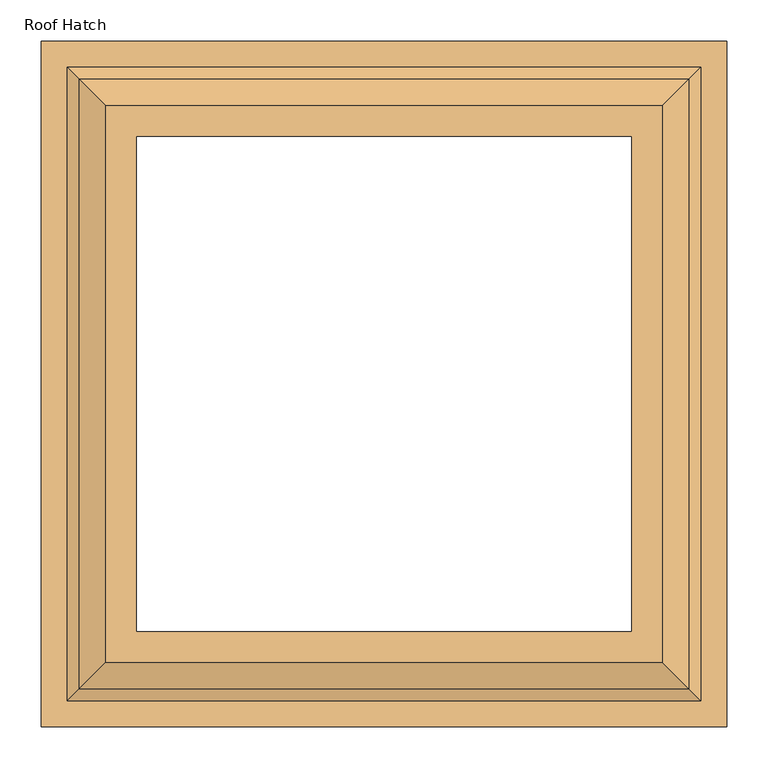
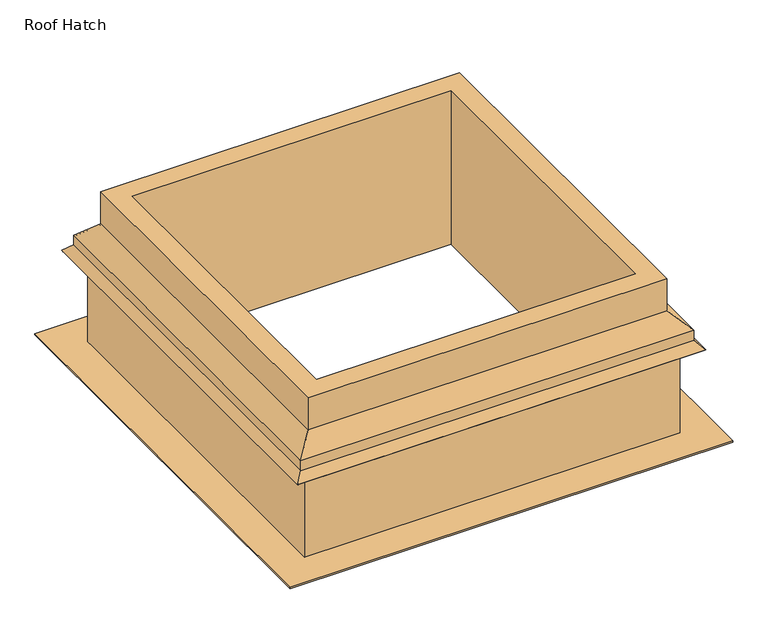
"""IFC4 building model written with IfcOpenShell, lengths in millimetres: door geometry, Alçap_o : Roof Hatch."""

import ifcopenshell
import ifcopenshell.guid

model = None  # the IFC model being written
_history = None  # IfcOwnerHistory: only IFC2X3 demands one
_inside = {}  # id of a spatial element -> (the spatial element, [elements in it])
_under = {}  # id of a project, library or spatial element -> (it, [spatial elements below it])
_declared = {}  # id of a project -> (the project, [libraries it declares])
_typed = {}  # id of a type object -> (the type object, [elements of that type])
_made_of = {}  # id of a material, layer set ... -> (it, [elements and type objects made of it])


def new_model(schema):
    """Start an empty IFC model of exactly this schema.

    Asked for "IFC4X3", IfcOpenShell would pick the latest addendum, in which some entities
    have other attributes; the version numbers below select the first issue.
    IFC2X3 requires an IfcOwnerHistory on every rooted entity: one is made here for all.
    """
    global model, _history
    if schema == "IFC4X3":
        model = ifcopenshell.file(schema_version=(4, 3, 0, 0))
    else:
        model = ifcopenshell.file(schema=schema)
    _inside.clear()
    _under.clear()
    _declared.clear()
    _typed.clear()
    _made_of.clear()
    _history = None
    if model.schema == "IFC2X3":
        org = make("IfcOrganization", Name="unknown")
        user = make(
            "IfcPersonAndOrganization",
            ThePerson=make("IfcPerson", FamilyName="unknown"),
            TheOrganization=org,
        )
        app = make(
            "IfcApplication",
            ApplicationDeveloper=org,
            Version="unknown",
            ApplicationFullName="unknown",
            ApplicationIdentifier="unknown",
        )
        _history = make(
            "IfcOwnerHistory",
            OwningUser=user,
            OwningApplication=app,
            ChangeAction="ADDED",
            CreationDate=0,
        )
    return model


def make(cls, **values):
    """One entity of the class cls with the attributes given. An attribute that is None is left unset."""
    return model.create_entity(
        cls, **{name: value for name, value in values.items() if value is not None}
    )


def rooted(cls, **values):
    """An entity with a GlobalId (a new one), such as an element, a storey or a relation."""
    return make(cls, GlobalId=ifcopenshell.guid.new(), OwnerHistory=_history, **values)


def si_unit(unit_type, name, prefix=None):
    """IfcSIUnit, for example si_unit("LENGTHUNIT", "METRE", prefix="MILLI")."""
    return make("IfcSIUnit", UnitType=unit_type, Prefix=prefix, Name=name)


def assignment(units):
    """IfcUnitAssignment: the units of a project."""
    return None if units is None else make("IfcUnitAssignment", Units=units)


def point(xyz):
    """IfcCartesianPoint."""
    return None if xyz is None else make("IfcCartesianPoint", Coordinates=xyz)


def direction(xyz):
    """IfcDirection."""
    return None if xyz is None else make("IfcDirection", DirectionRatios=xyz)


def frame(location, z_axis=None, x_axis=None):
    """IfcAxis2Placement3D, a coordinate frame: its origin and axes. An axis left out is left unset."""
    return make(
        "IfcAxis2Placement3D",
        Location=point(location),
        Axis=direction(z_axis),
        RefDirection=direction(x_axis),
    )


def origin():
    """The frame at (0, 0, 0) with its axes left unset."""
    return frame((0.0, 0.0, 0.0))


def place(relative_to, where):
    """IfcLocalPlacement: puts the frame where relative to a parent placement (None: the world)."""
    return make(
        "IfcLocalPlacement", PlacementRelTo=relative_to, RelativePlacement=where
    )


def context(
    kind, dimensions, precision=None, world=None, true_north=None, identifier=None
):
    """IfcGeometricRepresentationContext, for example the 3D "Model" context."""
    return make(
        "IfcGeometricRepresentationContext",
        ContextIdentifier=identifier,
        ContextType=kind,
        CoordinateSpaceDimension=dimensions,
        Precision=precision,
        WorldCoordinateSystem=world,
        TrueNorth=true_north,
    )


def project(units=None, contexts=None):
    """IfcProject with its units and contexts."""
    return rooted(
        "IfcProject",
        Name="project",
        RepresentationContexts=contexts,
        UnitsInContext=assignment(units),
    )


def spatial(cls, under=None, at=None, **own):
    """A site, building, storey or space (cls), placed at a placement, below another one or the project."""
    s = rooted(cls, ObjectPlacement=at, **own)
    if under is not None:
        _under.setdefault(under.id(), (under, []))[1].append(s)
    return s


def faces_of(points, faces, orient=None, outer=None):
    """IfcFace entities. A face is a list of loops; a loop is a list of indices into points, from 0.

    orient and outer hold one flag for each loop. By default every Orientation is true, the
    first loop of a face is its IfcFaceOuterBound and the others are IfcFaceBound.
    """
    made = []
    for i, loops in enumerate(faces):
        bounds = []
        for j, loop in enumerate(loops):
            is_outer = j == 0 if outer is None else outer[i][j]
            bounds.append(
                make(
                    "IfcFaceOuterBound" if is_outer else "IfcFaceBound",
                    Bound=make("IfcPolyLoop", Polygon=[points[k] for k in loop]),
                    Orientation=True if orient is None else orient[i][j],
                )
            )
        made.append(make("IfcFace", Bounds=bounds))
    return made


def faceted_brep(points, faces, orient=None, outer=None, voids=None):
    """IfcFacetedBrep: a solid bounded by flat faces; with voids (closed shells), ...WithVoids."""
    shared = [point(p) for p in points]
    hull = make("IfcClosedShell", CfsFaces=faces_of(shared, faces, orient, outer))
    if voids is None:
        return make("IfcFacetedBrep", Outer=hull)
    return make(
        "IfcFacetedBrepWithVoids",
        Outer=hull,
        Voids=[
            make(cls, CfsFaces=faces_of(shared, fs, o, b)) for cls, fs, o, b in voids
        ],
    )


def shape(context_of_items, identifier, shape_type, items):
    """IfcShapeRepresentation: the items that make up one representation, for example the "Body"."""
    return make(
        "IfcShapeRepresentation",
        ContextOfItems=context_of_items,
        RepresentationIdentifier=identifier,
        RepresentationType=shape_type,
        Items=items,
    )


def source(mapping_origin, context_of_items, identifier, shape_type, items):
    """IfcRepresentationMap: a shape defined once, which mapped items show again and again."""
    return make(
        "IfcRepresentationMap",
        MappingOrigin=mapping_origin,
        MappedRepresentation=shape(context_of_items, identifier, shape_type, items),
    )


def transform(
    local_origin,
    x_axis=None,
    y_axis=None,
    z_axis=None,
    scale=None,
    scale2=None,
    scale3=None,
    uniform=True,
):
    """IfcCartesianTransformationOperator3D, or its non-uniform kind. x_axis, y_axis, z_axis: its Axis1, 2, 3."""
    if uniform:
        return make(
            "IfcCartesianTransformationOperator3D",
            Axis1=direction(x_axis),
            Axis2=direction(y_axis),
            LocalOrigin=point(local_origin),
            Scale=scale,
            Axis3=direction(z_axis),
        )
    return make(
        "IfcCartesianTransformationOperator3DnonUniform",
        Axis1=direction(x_axis),
        Axis2=direction(y_axis),
        LocalOrigin=point(local_origin),
        Scale=scale,
        Axis3=direction(z_axis),
        Scale2=scale2,
        Scale3=scale3,
    )


def mapped(mapping_source, mapping_target):
    """IfcMappedItem: shows the shape of a source again, moved by a transform."""
    return make(
        "IfcMappedItem", MappingSource=mapping_source, MappingTarget=mapping_target
    )


def made_of(thing, what):
    """Note that an element or type object is made of a material, layer set ...; save() writes the relation."""
    if what is not None:
        _made_of.setdefault(what.id(), (what, []))[1].append(thing)
    return thing


def element(
    cls,
    number,
    at=None,
    inside=None,
    cuts=None,
    type_object=None,
    material=None,
    context=None,
    identifier="Body",
    shape_type=None,
    held_by="IfcProductDefinitionShape",
    body=None,
    shapes=None,
    **own,
):
    """One element of the class cls, such as IfcWall. Its Tag is "e" and its number.

    at: its placement. inside: the storey or other place that contains it. cuts: it is an
    opening in that element (IfcRelVoidsElement). A single representation is given by context,
    identifier, shape_type and body (its items); several are given by shapes. held_by: the class
    of the entity that holds the representations. save() writes the other relations.
    """
    e = rooted(cls, Tag="e%d" % number, ObjectPlacement=at, **own)
    if body is not None:
        shapes = [shape(context, identifier, shape_type, body)]
    if shapes is not None:
        e.Representation = make(held_by, Representations=shapes)
    if inside is not None:
        _inside.setdefault(inside.id(), (inside, []))[1].append(e)
    if cuts is not None:
        rooted(
            "IfcRelVoidsElement", RelatingBuildingElement=cuts, RelatedOpeningElement=e
        )
    if type_object is not None:
        _typed.setdefault(type_object.id(), (type_object, []))[1].append(e)
    return made_of(e, material)


def aggregate(whole, parts):
    """IfcRelAggregates: a whole, such as a stair, and the parts it consists of."""
    return rooted("IfcRelAggregates", RelatingObject=whole, RelatedObjects=parts)


def save(model, path):
    """Write the relations noted so far, then the file.

    IfcRelAggregates (storeys below a building ...), IfcRelContainedInSpatialStructure (elements
    in a storey), IfcRelDefinesByType, IfcRelAssociatesMaterial and IfcRelDeclares: one each for
    every whole, place, type object, material and project.
    """
    for whole, parts in _under.values():
        aggregate(whole, parts)
    for where, things in _inside.values():
        rooted(
            "IfcRelContainedInSpatialStructure",
            RelatedElements=things,
            RelatingStructure=where,
        )
    for kind, things in _typed.values():
        rooted("IfcRelDefinesByType", RelatedObjects=things, RelatingType=kind)
    for what, things in _made_of.values():
        rooted("IfcRelAssociatesMaterial", RelatedObjects=things, RelatingMaterial=what)
    for by, libraries in _declared.values():
        rooted("IfcRelDeclares", RelatingContext=by, RelatedDefinitions=libraries)
    model.write(path)


def roof_hatch_26298362(model_context):
    return source(origin(), model_context, "Body", "Brep", [
        faceted_brep([(119.78125, 353.18125, 2.38125), (119.78125, 353.18125, 224.63125), (119.78125, -353.18125, 224.63125), (119.78125, -353.18125, 2.38125), (68.98125, 302.38125, 230.98125), (68.98125, 302.38125, 2.38125), (68.98125, -302.38125, 2.38125), (68.98125, -302.38125, 230.98125), (-586.58125, -353.18125, 224.63125), (-586.58125, -353.18125, 2.38125), (-535.78125, -302.38125, 2.38125), (-535.78125, -302.38125, 230.98125), (-586.58125, 353.18125, 224.63125), (-586.58125, 353.18125, 2.38125), (-535.78125, 302.38125, 2.38125), (-535.78125, 302.38125, 230.98125), (113.43125, 346.83125, 230.98125), (-580.23125, 346.83125, 230.98125), (-580.23125, -346.83125, 230.98125), (113.43125, -346.83125, 230.98125)], [[[0, 1, 2, 3]], [[4, 5, 6, 7]], [[3, 2, 8, 9]], [[7, 6, 10, 11]], [[9, 8, 12, 13]], [[11, 10, 14, 15]], [[16, 17, 18, 19], [7, 11, 15, 4]], [[13, 12, 1, 0]], [[3, 9, 13, 0], [5, 14, 10, 6]], [[15, 14, 5, 4]], [[1, 16, 19, 2]], [[2, 19, 18, 8]], [[8, 18, 17, 12]], [[12, 17, 16, 1]]]),
        faceted_brep([(66.6, 300.0, 304.8), (66.6, 300.0, 0.0), (66.6, -300.0, 0.0), (66.6, -300.0, 304.8), (104.303125, 337.703125, 241.3), (104.303125, 337.703125, 304.8), (104.303125, -337.703125, 304.8), (104.303125, -337.703125, 241.3), (136.45, 369.85, 190.5), (136.45, 369.85, 210.1272727), (136.45, -369.85, 210.1272727), (136.45, -369.85, 190.5), (151.134375, 384.534375, 175.815625), (151.134375, -384.534375, 175.815625), (149.450577, 382.850577, 174.131827), (149.450577, -382.850577, 174.131827), (134.06875, 367.46875, 189.513654), (134.06875, -367.46875, 189.513654), (134.06875, 367.46875, 209.1193993), (134.06875, -367.46875, 209.1193993), (101.921875, 335.321875, 302.41875), (101.921875, 335.321875, 240.2921266), (101.921875, -335.321875, 240.2921266), (101.921875, -335.321875, 302.41875), (68.98125, 302.38125, 2.38125), (68.98125, 302.38125, 302.41875), (68.98125, -302.38125, 302.41875), (68.98125, -302.38125, 2.38125), (182.884375, 416.284375, 0.0), (182.884375, 416.284375, 2.38125), (182.884375, -416.284375, 2.38125), (182.884375, -416.284375, 0.0), (-533.4, -300.0, 0.0), (-533.4, -300.0, 304.8), (-571.103125, -337.703125, 304.8), (-571.103125, -337.703125, 241.3), (-603.25, -369.85, 210.1272727), (-603.25, -369.85, 190.5), (-617.934375, -384.534375, 175.815625), (-616.250577, -382.850577, 174.131827), (-600.86875, -367.46875, 189.513654), (-600.86875, -367.46875, 209.1193993), (-568.721875, -335.321875, 240.2921266), (-568.721875, -335.321875, 302.41875), (-535.78125, -302.38125, 302.41875), (-535.78125, -302.38125, 2.38125), (-649.684375, -416.284375, 2.38125), (-649.684375, -416.284375, 0.0), (-533.4, 300.0, 0.0), (-533.4, 300.0, 304.8), (-571.103125, 337.703125, 304.8), (-571.103125, 337.703125, 241.3), (-603.25, 369.85, 210.1272727), (-603.25, 369.85, 190.5), (-617.934375, 384.534375, 175.815625), (-616.250577, 382.850577, 174.131827), (-600.86875, 367.46875, 189.513654), (-600.86875, 367.46875, 209.1193993), (-568.721875, 335.321875, 240.2921266), (-568.721875, 335.321875, 302.41875), (-535.78125, 302.38125, 302.41875), (-535.78125, 302.38125, 2.38125), (-649.684375, 416.284375, 2.38125), (-649.684375, 416.284375, 0.0)], [[[0, 1, 2, 3]], [[4, 5, 6, 7]], [[8, 9, 10, 11]], [[12, 8, 11, 13]], [[14, 12, 13, 15]], [[16, 14, 15, 17]], [[18, 16, 17, 19]], [[20, 21, 22, 23]], [[24, 25, 26, 27]], [[28, 29, 30, 31]], [[3, 2, 32, 33]], [[7, 6, 34, 35]], [[11, 10, 36, 37]], [[13, 11, 37, 38]], [[15, 13, 38, 39]], [[17, 15, 39, 40]], [[19, 17, 40, 41]], [[23, 22, 42, 43]], [[27, 26, 44, 45]], [[31, 30, 46, 47]], [[33, 32, 48, 49]], [[35, 34, 50, 51]], [[37, 36, 52, 53]], [[38, 37, 53, 54]], [[39, 38, 54, 55]], [[40, 39, 55, 56]], [[41, 40, 56, 57]], [[43, 42, 58, 59]], [[45, 44, 60, 61]], [[47, 46, 62, 63]], [[49, 48, 1, 0]], [[5, 50, 34, 6], [3, 33, 49, 0]], [[51, 50, 5, 4]], [[53, 52, 9, 8]], [[54, 53, 8, 12]], [[55, 54, 12, 14]], [[56, 55, 14, 16]], [[57, 56, 16, 18]], [[59, 58, 21, 20]], [[23, 43, 59, 20], [25, 60, 44, 26]], [[61, 60, 25, 24]], [[29, 62, 46, 30], [27, 45, 61, 24]], [[63, 62, 29, 28]], [[31, 47, 63, 28], [1, 48, 32, 2]], [[9, 4, 7, 10]], [[21, 18, 19, 22]], [[10, 7, 35, 36]], [[22, 19, 41, 42]], [[36, 35, 51, 52]], [[42, 41, 57, 58]], [[52, 51, 4, 9]], [[58, 57, 18, 21]]]),
    ])


if __name__ == "__main__":
    model = new_model("IFC4")
    model_context = context("Model", 3, world=origin())
    ifc_project = project(units=[si_unit("LENGTHUNIT", "METRE", prefix="MILLI")], contexts=[model_context])
    site = spatial("IfcSite", under=ifc_project)
    building = spatial("IfcBuilding", under=site)
    placement = place(None, origin())
    roof_hatch_shape = roof_hatch_26298362(model_context)
    element("IfcDoor", 1, ObjectType="Alçap_o : Roof Hatch", at=placement, inside=building, context=model_context, shape_type="MappedRepresentation", body=[
        mapped(roof_hatch_shape, transform((0.0, 0.0, 0.0), x_axis=(1.0, 0.0, 0.0), y_axis=(0.0, 1.0, 0.0), z_axis=(0.0, 0.0, 1.0))),
    ])
    save(model, "model.ifc")

# Revit data of these elements
# Type "Alçap_o : Roof Hatch"
#   Type Mark = "P73"
#   Warranty = ""
#   URL Product = "http://www.bilco.com/foundations/store/shopdetail.asp?product=1S-1"
#   URL = "http://www.bilco.com/"
#   Analytic Construction = "<Nenhum>"
#   Release Date = ""
#   Observations = ""
#   Model = "Type S Roof Hatch"
#   Manufacturer = "Bilco"
#   Line = ""
#   Installation = ""
#   Industry Standards = ""
#   Designer = ""
#   Description = "Roof Hatch"
#   Date Maintenance = ""
#   Date Installation = ""
#   Customer Service Contact = ""
#   Created by = "Contino"
#   Certification = ""
#   Assembly Code = "B2030900"
#   Appoved by = "Contino"
#   Width = 0.600 m
#   Weight = 0
#   Rough Width = 0.6508 m
#   Rough Height = 0.6508 m
#   Length = 0.600 m
#   Height = 0.319881 m
#   Default Elevation = 1.2192 m
#   Cover Width = 0.73335 m
#   Cover Opening = 90.00°
#   Cover Length = 0.7016 m
#   Hatch Open [instance default] = yes
#   Hardware = Stainless Steel-Bilco-Sand Blast Finish-304
#   Gasket = Plastic-Bilco-Rubber Black
#   Frame = Stainless Steel-Bilco-Sand Blast Finish-304
#   Finish = Galvanized Steel - Bilco - Red Oxide Primer Finish
#   Fiberboard Insulation = Insulation-Bilco-Rigid Insulation
#   Dome = Plastic-Bilco-Polycarbonate
#   Cover = Galvanized Steel-Bilco-Red Oxide Primer Finish
#   Function = (empty or 0)
# Element 1 (IfcDoor, "Alçap_o : Roof Hatch")
#   Hatch Open = no
#   Materials on its faces: "Stainless Steel-Bilco-Sand Blast Finish-304", "Insulation-Bilco-Rigid Insulation"
# Materials
#   "Stainless Steel-Bilco-Sand Blast Finish-304": class "Metal", colour RGB 189 187 185, transparency 0, Manufacturer = "Add Manufacturer Name", URL = "Add Manufacturer URL", Cost = 0
#   "Plastic-Bilco-Rubber Black": class "Plastic", colour RGB 63 63 63, transparency 0, Manufacturer = "Add Manufacturer Name", URL = "Add Manufacturer URL", Cost = 0
#   "Galvanized Steel - Bilco - Red Oxide Primer Finish": class "Metal", colour RGB 160 81 45, transparency 0, Manufacturer = "Add Manufacturer Name", URL = "Add Manufacturer URL", Cost = 0
#   "Insulation-Bilco-Rigid Insulation": class "Miscellaneous", colour RGB 182 181 179, transparency 0
#   "Plastic-Bilco-Polycarbonate": class "Plastic", colour RGB 165 165 165, transparency 0.46, Cost = 0
#   "Galvanized Steel-Bilco-Red Oxide Primer Finish": class "Paint", colour RGB 160 81 45, transparency 0, Manufacturer = "Add Manufacturer Name", URL = "Add Manufacturer URL", Cost = 0
